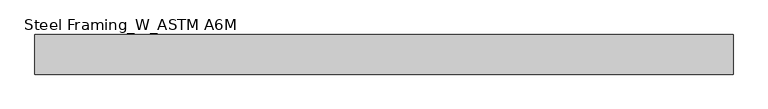
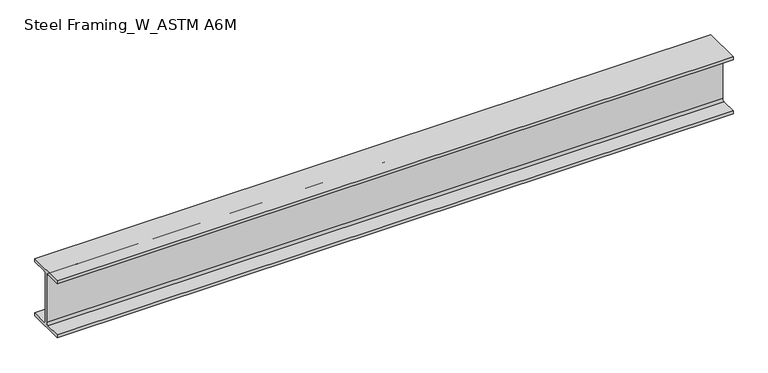
"""IFC4 building model written with IfcOpenShell, lengths in millimetres: beam geometry, Steel Framing_W_ASTM A6M : H_SB_AR_S02_W200x31.3_B6."""

import ifcopenshell
import ifcopenshell.guid

model = None  # the IFC model being written
_history = None  # IfcOwnerHistory: only IFC2X3 demands one
_inside = {}  # id of a spatial element -> (the spatial element, [elements in it])
_under = {}  # id of a project, library or spatial element -> (it, [spatial elements below it])
_declared = {}  # id of a project -> (the project, [libraries it declares])
_typed = {}  # id of a type object -> (the type object, [elements of that type])
_made_of = {}  # id of a material, layer set ... -> (it, [elements and type objects made of it])


def new_model(schema):
    """Start an empty IFC model of exactly this schema.

    Asked for "IFC4X3", IfcOpenShell would pick the latest addendum, in which some entities
    have other attributes; the version numbers below select the first issue.
    IFC2X3 requires an IfcOwnerHistory on every rooted entity: one is made here for all.
    """
    global model, _history
    if schema == "IFC4X3":
        model = ifcopenshell.file(schema_version=(4, 3, 0, 0))
    else:
        model = ifcopenshell.file(schema=schema)
    _inside.clear()
    _under.clear()
    _declared.clear()
    _typed.clear()
    _made_of.clear()
    _history = None
    if model.schema == "IFC2X3":
        org = make("IfcOrganization", Name="unknown")
        user = make(
            "IfcPersonAndOrganization",
            ThePerson=make("IfcPerson", FamilyName="unknown"),
            TheOrganization=org,
        )
        app = make(
            "IfcApplication",
            ApplicationDeveloper=org,
            Version="unknown",
            ApplicationFullName="unknown",
            ApplicationIdentifier="unknown",
        )
        _history = make(
            "IfcOwnerHistory",
            OwningUser=user,
            OwningApplication=app,
            ChangeAction="ADDED",
            CreationDate=0,
        )
    return model


def make(cls, **values):
    """One entity of the class cls with the attributes given. An attribute that is None is left unset."""
    return model.create_entity(
        cls, **{name: value for name, value in values.items() if value is not None}
    )


def rooted(cls, **values):
    """An entity with a GlobalId (a new one), such as an element, a storey or a relation."""
    return make(cls, GlobalId=ifcopenshell.guid.new(), OwnerHistory=_history, **values)


def si_unit(unit_type, name, prefix=None):
    """IfcSIUnit, for example si_unit("LENGTHUNIT", "METRE", prefix="MILLI")."""
    return make("IfcSIUnit", UnitType=unit_type, Prefix=prefix, Name=name)


def assignment(units):
    """IfcUnitAssignment: the units of a project."""
    return None if units is None else make("IfcUnitAssignment", Units=units)


def point(xyz):
    """IfcCartesianPoint."""
    return None if xyz is None else make("IfcCartesianPoint", Coordinates=xyz)


def direction(xyz):
    """IfcDirection."""
    return None if xyz is None else make("IfcDirection", DirectionRatios=xyz)


def frame(location, z_axis=None, x_axis=None):
    """IfcAxis2Placement3D, a coordinate frame: its origin and axes. An axis left out is left unset."""
    return make(
        "IfcAxis2Placement3D",
        Location=point(location),
        Axis=direction(z_axis),
        RefDirection=direction(x_axis),
    )


def frame_2d(location, x_axis=None):
    """IfcAxis2Placement2D, a coordinate frame in the plane: its origin and x axis."""
    return make(
        "IfcAxis2Placement2D", Location=point(location), RefDirection=direction(x_axis)
    )


def origin():
    """The frame at (0, 0, 0) with its axes left unset."""
    return frame((0.0, 0.0, 0.0))


def place(relative_to, where):
    """IfcLocalPlacement: puts the frame where relative to a parent placement (None: the world)."""
    return make(
        "IfcLocalPlacement", PlacementRelTo=relative_to, RelativePlacement=where
    )


def context(
    kind, dimensions, precision=None, world=None, true_north=None, identifier=None
):
    """IfcGeometricRepresentationContext, for example the 3D "Model" context."""
    return make(
        "IfcGeometricRepresentationContext",
        ContextIdentifier=identifier,
        ContextType=kind,
        CoordinateSpaceDimension=dimensions,
        Precision=precision,
        WorldCoordinateSystem=world,
        TrueNorth=true_north,
    )


def project(units=None, contexts=None):
    """IfcProject with its units and contexts."""
    return rooted(
        "IfcProject",
        Name="project",
        RepresentationContexts=contexts,
        UnitsInContext=assignment(units),
    )


def spatial(cls, under=None, at=None, **own):
    """A site, building, storey or space (cls), placed at a placement, below another one or the project."""
    s = rooted(cls, ObjectPlacement=at, **own)
    if under is not None:
        _under.setdefault(under.id(), (under, []))[1].append(s)
    return s


def polyline(points):
    """IfcPolyline through the points."""
    return make("IfcPolyline", Points=[point(p) for p in points])


def circle_curve(where, radius):
    """IfcCircle in the frame where."""
    return make("IfcCircle", Position=where, Radius=radius)


def trimmed(basis, trim1, trim2, sense, master):
    """IfcTrimmedCurve: the piece of a basis curve between two trims."""
    return make(
        "IfcTrimmedCurve",
        BasisCurve=basis,
        Trim1=trim1,
        Trim2=trim2,
        SenseAgreement=sense,
        MasterRepresentation=master,
    )


def segment(curve, same_sense, transition):
    """IfcCompositeCurveSegment."""
    return make(
        "IfcCompositeCurveSegment",
        Transition=transition,
        SameSense=same_sense,
        ParentCurve=curve,
    )


def composite_curve(segments, self_intersect=None):
    """IfcCompositeCurve: segments joined end to end."""
    return make("IfcCompositeCurve", Segments=segments, SelfIntersect=self_intersect)


def outline(outer, holes=None, kind="AREA"):
    """IfcArbitraryClosedProfileDef: a profile drawn as a closed curve; with holes, ...WithVoids."""
    if holes is None:
        return make("IfcArbitraryClosedProfileDef", ProfileType=kind, OuterCurve=outer)
    return make(
        "IfcArbitraryProfileDefWithVoids",
        ProfileType=kind,
        OuterCurve=outer,
        InnerCurves=holes,
    )


def extrude(swept, where, along, depth):
    """IfcExtrudedAreaSolid: the profile swept, set in the frame where, extruded along a direction by depth."""
    return make(
        "IfcExtrudedAreaSolid",
        SweptArea=swept,
        Position=where,
        ExtrudedDirection=direction(along),
        Depth=depth,
    )


def shape(context_of_items, identifier, shape_type, items):
    """IfcShapeRepresentation: the items that make up one representation, for example the "Body"."""
    return make(
        "IfcShapeRepresentation",
        ContextOfItems=context_of_items,
        RepresentationIdentifier=identifier,
        RepresentationType=shape_type,
        Items=items,
    )


def source(mapping_origin, context_of_items, identifier, shape_type, items):
    """IfcRepresentationMap: a shape defined once, which mapped items show again and again."""
    return make(
        "IfcRepresentationMap",
        MappingOrigin=mapping_origin,
        MappedRepresentation=shape(context_of_items, identifier, shape_type, items),
    )


def transform(
    local_origin,
    x_axis=None,
    y_axis=None,
    z_axis=None,
    scale=None,
    scale2=None,
    scale3=None,
    uniform=True,
):
    """IfcCartesianTransformationOperator3D, or its non-uniform kind. x_axis, y_axis, z_axis: its Axis1, 2, 3."""
    if uniform:
        return make(
            "IfcCartesianTransformationOperator3D",
            Axis1=direction(x_axis),
            Axis2=direction(y_axis),
            LocalOrigin=point(local_origin),
            Scale=scale,
            Axis3=direction(z_axis),
        )
    return make(
        "IfcCartesianTransformationOperator3DnonUniform",
        Axis1=direction(x_axis),
        Axis2=direction(y_axis),
        LocalOrigin=point(local_origin),
        Scale=scale,
        Axis3=direction(z_axis),
        Scale2=scale2,
        Scale3=scale3,
    )


def mapped(mapping_source, mapping_target):
    """IfcMappedItem: shows the shape of a source again, moved by a transform."""
    return make(
        "IfcMappedItem", MappingSource=mapping_source, MappingTarget=mapping_target
    )


def made_of(thing, what):
    """Note that an element or type object is made of a material, layer set ...; save() writes the relation."""
    if what is not None:
        _made_of.setdefault(what.id(), (what, []))[1].append(thing)
    return thing


def element(
    cls,
    number,
    at=None,
    inside=None,
    cuts=None,
    type_object=None,
    material=None,
    context=None,
    identifier="Body",
    shape_type=None,
    held_by="IfcProductDefinitionShape",
    body=None,
    shapes=None,
    **own,
):
    """One element of the class cls, such as IfcWall. Its Tag is "e" and its number.

    at: its placement. inside: the storey or other place that contains it. cuts: it is an
    opening in that element (IfcRelVoidsElement). A single representation is given by context,
    identifier, shape_type and body (its items); several are given by shapes. held_by: the class
    of the entity that holds the representations. save() writes the other relations.
    """
    e = rooted(cls, Tag="e%d" % number, ObjectPlacement=at, **own)
    if body is not None:
        shapes = [shape(context, identifier, shape_type, body)]
    if shapes is not None:
        e.Representation = make(held_by, Representations=shapes)
    if inside is not None:
        _inside.setdefault(inside.id(), (inside, []))[1].append(e)
    if cuts is not None:
        rooted(
            "IfcRelVoidsElement", RelatingBuildingElement=cuts, RelatedOpeningElement=e
        )
    if type_object is not None:
        _typed.setdefault(type_object.id(), (type_object, []))[1].append(e)
    return made_of(e, material)


def aggregate(whole, parts):
    """IfcRelAggregates: a whole, such as a stair, and the parts it consists of."""
    return rooted("IfcRelAggregates", RelatingObject=whole, RelatedObjects=parts)


def save(model, path):
    """Write the relations noted so far, then the file.

    IfcRelAggregates (storeys below a building ...), IfcRelContainedInSpatialStructure (elements
    in a storey), IfcRelDefinesByType, IfcRelAssociatesMaterial and IfcRelDeclares: one each for
    every whole, place, type object, material and project.
    """
    for whole, parts in _under.values():
        aggregate(whole, parts)
    for where, things in _inside.values():
        rooted(
            "IfcRelContainedInSpatialStructure",
            RelatedElements=things,
            RelatingStructure=where,
        )
    for kind, things in _typed.values():
        rooted("IfcRelDefinesByType", RelatedObjects=things, RelatingType=kind)
    for what, things in _made_of.values():
        rooted("IfcRelAssociatesMaterial", RelatedObjects=things, RelatingMaterial=what)
    for by, libraries in _declared.values():
        rooted("IfcRelDeclares", RelatingContext=by, RelatedDefinitions=libraries)
    model.write(path)


def steel_framing_w_astm_a6m_0c2b25f3(model_context):
    return source(origin(), model_context, "Body", "SweptSolid", [
        extrude(outline(composite_curve([segment(polyline([(67.0, -94.8), (67.0, -105.0), (-67.0, -105.0), (-67.0, -94.8), (-10.775, -94.8)]), True, "CONTINUOUS"), segment(trimmed(circle_curve(frame_2d((-10.775, -87.2)), 7.6), [point((-10.775, -94.8))], [point((-3.175, -87.2))], True, "CARTESIAN"), True, "CONTINUOUS"), segment(polyline([(-3.175, -87.2), (-3.175, 87.2)]), True, "CONTINUOUS"), segment(trimmed(circle_curve(frame_2d((-10.775, 87.2)), 7.6), [point((-3.175, 87.2))], [point((-10.775, 94.8))], True, "CARTESIAN"), True, "CONTINUOUS"), segment(polyline([(-10.775, 94.8), (-67.0, 94.8), (-67.0, 105.0), (67.0, 105.0), (67.0, 94.8), (10.775, 94.8)]), True, "CONTINUOUS"), segment(trimmed(circle_curve(frame_2d((10.775, 87.2)), 7.6), [point((10.775, 94.8))], [point((3.175, 87.2))], True, "CARTESIAN"), True, "CONTINUOUS"), segment(polyline([(3.175, 87.2), (3.175, -87.2)]), True, "CONTINUOUS"), segment(trimmed(circle_curve(frame_2d((10.775, -87.2)), 7.6), [point((3.175, -87.2))], [point((10.775, -94.8))], True, "CARTESIAN"), True, "CONTINUOUS"), segment(polyline([(10.775, -94.8), (67.0, -94.8)]), True, "CONTINUOUS")], self_intersect=False)), frame((-1181.3, 0.0, 0.0), z_axis=(1.0, 0.0, 0.0), x_axis=(0.0, 1.0, 0.0)), (0.0, 0.0, 1.0), 2362.6),
    ])


if __name__ == "__main__":
    model = new_model("IFC4")
    model_context = context("Model", 3, world=origin())
    ifc_project = project(units=[si_unit("LENGTHUNIT", "METRE", prefix="MILLI")], contexts=[model_context])
    site = spatial("IfcSite", under=ifc_project)
    building = spatial("IfcBuilding", under=site)
    placement = place(None, origin())
    steel_framing_w_astm_a6m_shape = steel_framing_w_astm_a6m_0c2b25f3(model_context)
    element("IfcBeam", 1, ObjectType="Steel Framing_W_ASTM A6M : H_SB_AR_S02_W200x31.3_B6", at=placement, inside=building, context=model_context, shape_type="MappedRepresentation", body=[
        mapped(steel_framing_w_astm_a6m_shape, transform((0.0, 0.0, 0.0), x_axis=(1.0, 0.0, 0.0), y_axis=(0.0, 1.0, 0.0), z_axis=(0.0, 0.0, 1.0))),
    ])
    save(model, "model.ifc")

# Revit data of these elements
# Type "Steel Framing_W_ASTM A6M : H_SB_AR_S02_W200x31.3_B6"
#   Type Mark = "B6"
#   Section Name Key = "W8x21"
#   Width = 13.4 cm
#   Web Thickness = 0.635 cm
#   Web Fillet = 0.76 cm
#   Warping Constant = 40800.0 cm⁶
#   Torsional Moment of Inertia = 11.70 cm⁴
#   Section Area = 39.7 cm²
#   Plastic Modulus weak axis = 93.2 cm³
#   Plastic Modulus strong axis = 334.0 cm³
#   Perimeter = 0.93 m²/m
#   Nominal Weight = 31.30 kgf/m
#   Moment of Inertia weak axis = 407.00 cm⁴
#   Moment of Inertia strong axis = 3130.00 cm⁴
#   Height = 21.0 cm
#   Flange Thickness = 1.02 cm
#   Elastic Modulus weak axis = 60.8 cm³
#   Elastic Modulus strong axis = 298.0 cm³
#   Centroid Vertical = 10.5 cm
#   Centroid Horizontal = 6.7 cm
#   Length [instance default] = 1500 mm
#   Structural Material [instance default] = Steel, 45-345
#   Bolt Spacing = 0
#   Assembly Code = ""
# Element 1 (IfcBeam, "Steel Framing_W_ASTM A6M : H_SB_AR_S02_W200x31.3_B6")
#   Materials on its faces: "Steel, 45-345"
# Materials
#   "Steel, 45-345": class "Metal", colour RGB 189 187 185, transparency 0, Description = "Steel 345 MPa", Cost = 0
